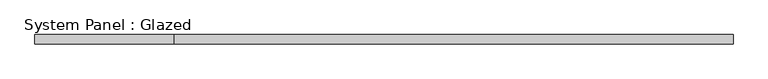
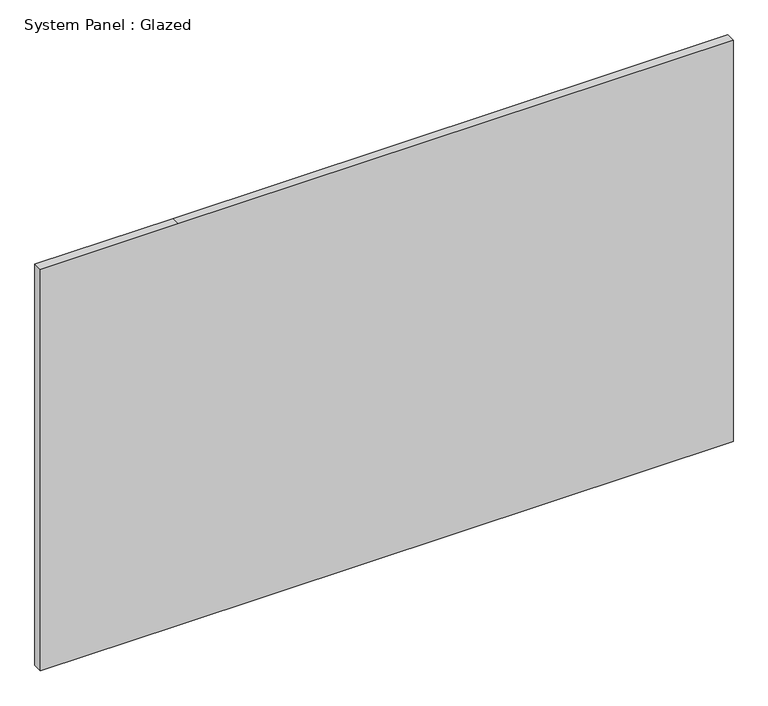
"""IFC4 building model written with IfcOpenShell, lengths in millimetres: plate geometry, System Panel : Glazed."""

import ifcopenshell
import ifcopenshell.guid

model = None  # the IFC model being written
_history = None  # IfcOwnerHistory: only IFC2X3 demands one
_inside = {}  # id of a spatial element -> (the spatial element, [elements in it])
_under = {}  # id of a project, library or spatial element -> (it, [spatial elements below it])
_declared = {}  # id of a project -> (the project, [libraries it declares])
_typed = {}  # id of a type object -> (the type object, [elements of that type])
_made_of = {}  # id of a material, layer set ... -> (it, [elements and type objects made of it])


def new_model(schema):
    """Start an empty IFC model of exactly this schema.

    Asked for "IFC4X3", IfcOpenShell would pick the latest addendum, in which some entities
    have other attributes; the version numbers below select the first issue.
    IFC2X3 requires an IfcOwnerHistory on every rooted entity: one is made here for all.
    """
    global model, _history
    if schema == "IFC4X3":
        model = ifcopenshell.file(schema_version=(4, 3, 0, 0))
    else:
        model = ifcopenshell.file(schema=schema)
    _inside.clear()
    _under.clear()
    _declared.clear()
    _typed.clear()
    _made_of.clear()
    _history = None
    if model.schema == "IFC2X3":
        org = make("IfcOrganization", Name="unknown")
        user = make(
            "IfcPersonAndOrganization",
            ThePerson=make("IfcPerson", FamilyName="unknown"),
            TheOrganization=org,
        )
        app = make(
            "IfcApplication",
            ApplicationDeveloper=org,
            Version="unknown",
            ApplicationFullName="unknown",
            ApplicationIdentifier="unknown",
        )
        _history = make(
            "IfcOwnerHistory",
            OwningUser=user,
            OwningApplication=app,
            ChangeAction="ADDED",
            CreationDate=0,
        )
    return model


def make(cls, **values):
    """One entity of the class cls with the attributes given. An attribute that is None is left unset."""
    return model.create_entity(
        cls, **{name: value for name, value in values.items() if value is not None}
    )


def rooted(cls, **values):
    """An entity with a GlobalId (a new one), such as an element, a storey or a relation."""
    return make(cls, GlobalId=ifcopenshell.guid.new(), OwnerHistory=_history, **values)


def si_unit(unit_type, name, prefix=None):
    """IfcSIUnit, for example si_unit("LENGTHUNIT", "METRE", prefix="MILLI")."""
    return make("IfcSIUnit", UnitType=unit_type, Prefix=prefix, Name=name)


def assignment(units):
    """IfcUnitAssignment: the units of a project."""
    return None if units is None else make("IfcUnitAssignment", Units=units)


def point(xyz):
    """IfcCartesianPoint."""
    return None if xyz is None else make("IfcCartesianPoint", Coordinates=xyz)


def direction(xyz):
    """IfcDirection."""
    return None if xyz is None else make("IfcDirection", DirectionRatios=xyz)


def frame(location, z_axis=None, x_axis=None):
    """IfcAxis2Placement3D, a coordinate frame: its origin and axes. An axis left out is left unset."""
    return make(
        "IfcAxis2Placement3D",
        Location=point(location),
        Axis=direction(z_axis),
        RefDirection=direction(x_axis),
    )


def origin():
    """The frame at (0, 0, 0) with its axes left unset."""
    return frame((0.0, 0.0, 0.0))


def place(relative_to, where):
    """IfcLocalPlacement: puts the frame where relative to a parent placement (None: the world)."""
    return make(
        "IfcLocalPlacement", PlacementRelTo=relative_to, RelativePlacement=where
    )


def context(
    kind, dimensions, precision=None, world=None, true_north=None, identifier=None
):
    """IfcGeometricRepresentationContext, for example the 3D "Model" context."""
    return make(
        "IfcGeometricRepresentationContext",
        ContextIdentifier=identifier,
        ContextType=kind,
        CoordinateSpaceDimension=dimensions,
        Precision=precision,
        WorldCoordinateSystem=world,
        TrueNorth=true_north,
    )


def project(units=None, contexts=None):
    """IfcProject with its units and contexts."""
    return rooted(
        "IfcProject",
        Name="project",
        RepresentationContexts=contexts,
        UnitsInContext=assignment(units),
    )


def spatial(cls, under=None, at=None, **own):
    """A site, building, storey or space (cls), placed at a placement, below another one or the project."""
    s = rooted(cls, ObjectPlacement=at, **own)
    if under is not None:
        _under.setdefault(under.id(), (under, []))[1].append(s)
    return s


def polyline(points):
    """IfcPolyline through the points."""
    return make("IfcPolyline", Points=[point(p) for p in points])


def outline(outer, holes=None, kind="AREA"):
    """IfcArbitraryClosedProfileDef: a profile drawn as a closed curve; with holes, ...WithVoids."""
    if holes is None:
        return make("IfcArbitraryClosedProfileDef", ProfileType=kind, OuterCurve=outer)
    return make(
        "IfcArbitraryProfileDefWithVoids",
        ProfileType=kind,
        OuterCurve=outer,
        InnerCurves=holes,
    )


def extrude(swept, where, along, depth):
    """IfcExtrudedAreaSolid: the profile swept, set in the frame where, extruded along a direction by depth."""
    return make(
        "IfcExtrudedAreaSolid",
        SweptArea=swept,
        Position=where,
        ExtrudedDirection=direction(along),
        Depth=depth,
    )


def shape(context_of_items, identifier, shape_type, items):
    """IfcShapeRepresentation: the items that make up one representation, for example the "Body"."""
    return make(
        "IfcShapeRepresentation",
        ContextOfItems=context_of_items,
        RepresentationIdentifier=identifier,
        RepresentationType=shape_type,
        Items=items,
    )


def source(mapping_origin, context_of_items, identifier, shape_type, items):
    """IfcRepresentationMap: a shape defined once, which mapped items show again and again."""
    return make(
        "IfcRepresentationMap",
        MappingOrigin=mapping_origin,
        MappedRepresentation=shape(context_of_items, identifier, shape_type, items),
    )


def transform(
    local_origin,
    x_axis=None,
    y_axis=None,
    z_axis=None,
    scale=None,
    scale2=None,
    scale3=None,
    uniform=True,
):
    """IfcCartesianTransformationOperator3D, or its non-uniform kind. x_axis, y_axis, z_axis: its Axis1, 2, 3."""
    if uniform:
        return make(
            "IfcCartesianTransformationOperator3D",
            Axis1=direction(x_axis),
            Axis2=direction(y_axis),
            LocalOrigin=point(local_origin),
            Scale=scale,
            Axis3=direction(z_axis),
        )
    return make(
        "IfcCartesianTransformationOperator3DnonUniform",
        Axis1=direction(x_axis),
        Axis2=direction(y_axis),
        LocalOrigin=point(local_origin),
        Scale=scale,
        Axis3=direction(z_axis),
        Scale2=scale2,
        Scale3=scale3,
    )


def mapped(mapping_source, mapping_target):
    """IfcMappedItem: shows the shape of a source again, moved by a transform."""
    return make(
        "IfcMappedItem", MappingSource=mapping_source, MappingTarget=mapping_target
    )


def made_of(thing, what):
    """Note that an element or type object is made of a material, layer set ...; save() writes the relation."""
    if what is not None:
        _made_of.setdefault(what.id(), (what, []))[1].append(thing)
    return thing


def element(
    cls,
    number,
    at=None,
    inside=None,
    cuts=None,
    type_object=None,
    material=None,
    context=None,
    identifier="Body",
    shape_type=None,
    held_by="IfcProductDefinitionShape",
    body=None,
    shapes=None,
    **own,
):
    """One element of the class cls, such as IfcWall. Its Tag is "e" and its number.

    at: its placement. inside: the storey or other place that contains it. cuts: it is an
    opening in that element (IfcRelVoidsElement). A single representation is given by context,
    identifier, shape_type and body (its items); several are given by shapes. held_by: the class
    of the entity that holds the representations. save() writes the other relations.
    """
    e = rooted(cls, Tag="e%d" % number, ObjectPlacement=at, **own)
    if body is not None:
        shapes = [shape(context, identifier, shape_type, body)]
    if shapes is not None:
        e.Representation = make(held_by, Representations=shapes)
    if inside is not None:
        _inside.setdefault(inside.id(), (inside, []))[1].append(e)
    if cuts is not None:
        rooted(
            "IfcRelVoidsElement", RelatingBuildingElement=cuts, RelatedOpeningElement=e
        )
    if type_object is not None:
        _typed.setdefault(type_object.id(), (type_object, []))[1].append(e)
    return made_of(e, material)


def aggregate(whole, parts):
    """IfcRelAggregates: a whole, such as a stair, and the parts it consists of."""
    return rooted("IfcRelAggregates", RelatingObject=whole, RelatedObjects=parts)


def save(model, path):
    """Write the relations noted so far, then the file.

    IfcRelAggregates (storeys below a building ...), IfcRelContainedInSpatialStructure (elements
    in a storey), IfcRelDefinesByType, IfcRelAssociatesMaterial and IfcRelDeclares: one each for
    every whole, place, type object, material and project.
    """
    for whole, parts in _under.values():
        aggregate(whole, parts)
    for where, things in _inside.values():
        rooted(
            "IfcRelContainedInSpatialStructure",
            RelatedElements=things,
            RelatingStructure=where,
        )
    for kind, things in _typed.values():
        rooted("IfcRelDefinesByType", RelatedObjects=things, RelatingType=kind)
    for what, things in _made_of.values():
        rooted("IfcRelAssociatesMaterial", RelatedObjects=things, RelatingMaterial=what)
    for by, libraries in _declared.values():
        rooted("IfcRelDeclares", RelatingContext=by, RelatedDefinitions=libraries)
    model.write(path)


def system_panel_glazed_1ad7f91b(model_context):
    return source(origin(), model_context, "Body", "SweptSolid", [
        extrude(outline(polyline([(0.0, -932.5428571), (0.0, -560.6142857), (0.0, 932.5428571), (1143.0, 932.5428571), (1143.0, -560.6142857), (1143.0, -932.5428571), (0.0, -932.5428571)])), frame((0.0, -12.7, 0.0), z_axis=(0.0, 1.0, 0.0), x_axis=(0.0, 0.0, 1.0)), (0.0, 0.0, 1.0), 25.4),
    ])


if __name__ == "__main__":
    model = new_model("IFC4")
    model_context = context("Model", 3, world=origin())
    ifc_project = project(units=[si_unit("LENGTHUNIT", "METRE", prefix="MILLI")], contexts=[model_context])
    site = spatial("IfcSite", under=ifc_project)
    building = spatial("IfcBuilding", under=site)
    placement = place(None, origin())
    system_panel_glazed_shape = system_panel_glazed_1ad7f91b(model_context)
    element("IfcPlate", 1, ObjectType="System Panel : Glazed", at=placement, inside=building, context=model_context, shape_type="MappedRepresentation", body=[
        mapped(system_panel_glazed_shape, transform((0.0, 0.0, 0.0), x_axis=(1.0, 0.0, 0.0), y_axis=(0.0, 1.0, 0.0), z_axis=(0.0, 0.0, 1.0))),
    ])
    save(model, "model.ifc")

# Revit data of these elements
# Element 1 (IfcPlate, "System Panel : Glazed")
#   Materials on its faces: "TEMPERED SAFETY GLAZING"
# Materials
#   "TEMPERED SAFETY GLAZING": class "Glass", colour RGB 236 240 239, transparency 0.41, Description = "Soda Lime Glass", Cost = 0
